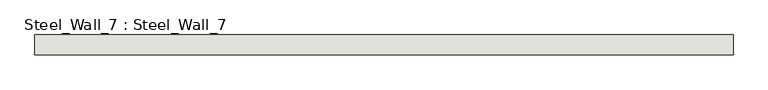
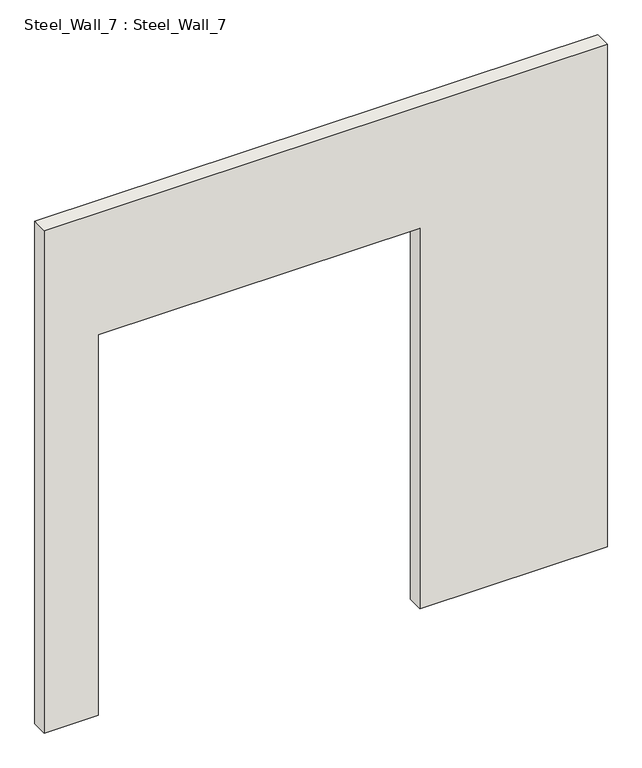
"""IFC4 building model written with IfcOpenShell, lengths in millimetres: wall geometry, Steel_Wall_7 : Steel_Wall_7."""

from ifc_helpers import new_model, si_unit, frame, origin, place, context, project, spatial, polyline, outline, extrude, source, transform, mapped, element, save


def steel_wall_7_steel_wall_7_8661bafb(model_context):
    return source(origin(), model_context, "Body", "SweptSolid", [
        extrude(outline(polyline([(3550.0, 6175.0), (3550.0, 2675.0), (250.0, 2675.0), (250.0, 3010.0), (2750.0, 3010.0), (2750.0, 5010.0), (250.0, 5010.0), (250.0, 6175.0), (3550.0, 6175.0)])), frame((0.0, 16755.0, 0.0), z_axis=(0.0, 1.0, 0.0), x_axis=(0.0, 0.0, 1.0)), (0.0, 0.0, 1.0), 100.0),
    ])


if __name__ == "__main__":
    model = new_model("IFC4")
    model_context = context("Model", 3, world=origin())
    ifc_project = project(units=[si_unit("LENGTHUNIT", "METRE", prefix="MILLI")], contexts=[model_context])
    site = spatial("IfcSite", under=ifc_project)
    building = spatial("IfcBuilding", under=site)
    placement = place(None, origin())
    steel_wall_7_steel_wall_7_shape = steel_wall_7_steel_wall_7_8661bafb(model_context)
    element("IfcWall", 1, ObjectType="Steel_Wall_7 : Steel_Wall_7", at=placement, inside=building, context=model_context, shape_type="MappedRepresentation", body=[
        mapped(steel_wall_7_steel_wall_7_shape, transform((0.0, 0.0, 0.0), x_axis=(1.0, 0.0, 0.0), y_axis=(0.0, 1.0, 0.0), z_axis=(0.0, 0.0, 1.0))),
    ])
    save(model, "model.ifc")

# Revit data of these elements
# Type "Steel_Wall_7 : Steel_Wall_7"
#   NameOverride = "Steel_Wall_7"
# Element 1 (IfcWall, "Steel_Wall_7 : Steel_Wall_7")
#   Materials on its faces: "IfcSurfaceStyle #33"
# Materials
#   "IfcSurfaceStyle #33": class "Unassigned", colour RGB 214 214 214, transparency 0
